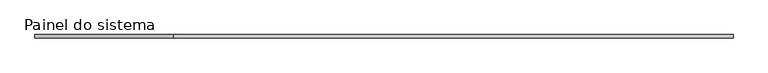
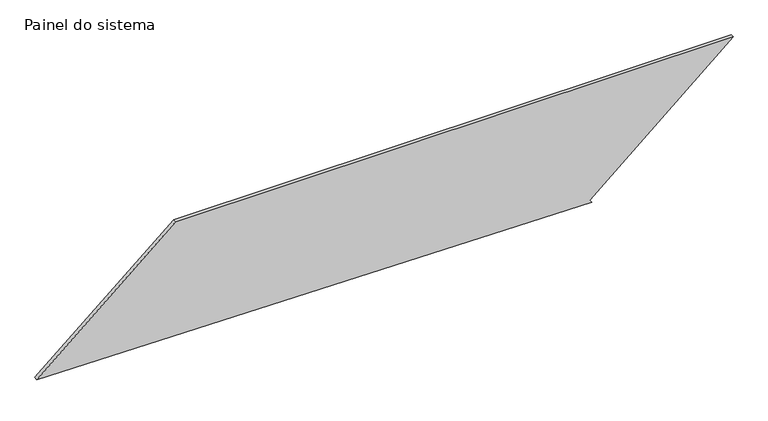
"""IFC4 building model written with IfcOpenShell, lengths in millimetres: plate geometry, Painel do sistema : Envidraçado."""

from ifc_helpers import new_model, si_unit, frame, origin, place, context, project, spatial, polyline, outline, extrude, source, transform, mapped, element, save


def painel_do_sistema_df117674(model_context):
    return source(origin(), model_context, "Body", "SweptSolid", [
        extrude(outline(polyline([(0.0, 1455.4316888), (19.0100862, 1439.1954139), (881.7100057, 2449.2793091), (881.7100057, -1473.4630767), (48.277665, -2449.2793091), (0.0, 1455.4316888)])), frame((0.0, 24.5, 0.0), z_axis=(0.0, 1.0, 0.0), x_axis=(0.0, 0.0, 1.0)), (0.0, 0.0, 1.0), 25.0),
    ])


if __name__ == "__main__":
    model = new_model("IFC4")
    model_context = context("Model", 3, world=origin())
    ifc_project = project(units=[si_unit("LENGTHUNIT", "METRE", prefix="MILLI")], contexts=[model_context])
    site = spatial("IfcSite", under=ifc_project)
    building = spatial("IfcBuilding", under=site)
    placement = place(None, origin())
    painel_do_sistema_shape = painel_do_sistema_df117674(model_context)
    element("IfcPlate", 1, ObjectType="Painel do sistema : Envidraçado", at=placement, inside=building, context=model_context, shape_type="MappedRepresentation", body=[
        mapped(painel_do_sistema_shape, transform((0.0, 0.0, 0.0), x_axis=(1.0, 0.0, 0.0), y_axis=(0.0, 1.0, 0.0), z_axis=(0.0, 0.0, 1.0))),
    ])
    save(model, "model.ifc")

# Revit data of these elements
# Type "Painel do sistema : Envidraçado"
#   Construction Type Id = "GSP4R"
#   Analytic Construction = "Vidraça única Pilkington 1/8 pol"
#   Visual Light Transmittance = 0.9
#   Solar Heat Gain Coefficient = 0.86
#   Heat Transfer Coefficient (U) = 6.7069 W/(m²·K)
# Element 1 (IfcPlate, "Painel do sistema : Envidraçado")
#   Materials on its faces: "Vidro"
# Materials
#   "Vidro": class "Vidro", colour RGB 0 128 192, transparency 0.9, Description = "Vidro de sílica", Cost = 0
